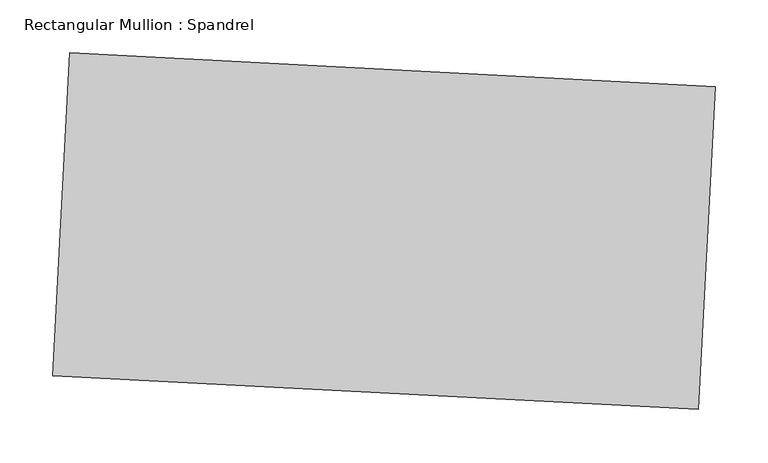
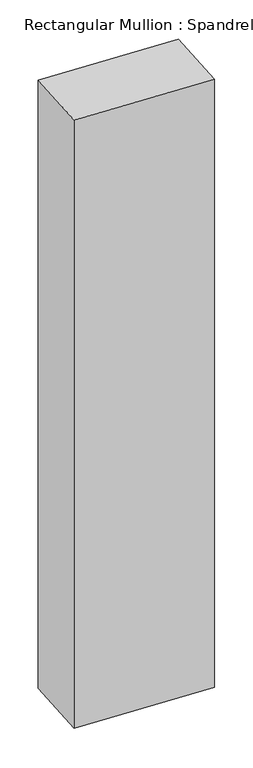
"""IFC4 building model written with IfcOpenShell, lengths in millimetres: member geometry, Rectangular Mullion : Spandrel."""

from ifc_helpers import new_model, si_unit, frame, origin, place, context, project, spatial, polyline, outline, extrude, source, transform, mapped, element, save


def rectangular_mullion_spandrel_2c0fee7e(model_context):
    return source(origin(), model_context, "Body", "SweptSolid", [
        extrude(outline(polyline([(7.5582819, 136.2391416), (-8.3937175, -168.1431406), (-617.1582819, -136.2391416), (-601.2062825, 168.1431406), (7.5582819, 136.2391416)])), frame((0.0, 0.0, -2875.2688367), z_axis=(0.0, 0.0, 1.0), x_axis=(1.0, 0.0, 0.0)), (0.0, 0.0, 1.0), 2875.2688367),
    ])


if __name__ == "__main__":
    model = new_model("IFC4")
    model_context = context("Model", 3, world=origin())
    ifc_project = project(units=[si_unit("LENGTHUNIT", "METRE", prefix="MILLI")], contexts=[model_context])
    site = spatial("IfcSite", under=ifc_project)
    building = spatial("IfcBuilding", under=site)
    placement = place(None, origin())
    rectangular_mullion_spandrel_shape = rectangular_mullion_spandrel_2c0fee7e(model_context)
    element("IfcMember", 1, ObjectType="Rectangular Mullion : Spandrel", at=placement, inside=building, context=model_context, shape_type="MappedRepresentation", body=[
        mapped(rectangular_mullion_spandrel_shape, transform((0.0, 0.0, 0.0), x_axis=(1.0, 0.0, 0.0), y_axis=(0.0, 1.0, 0.0), z_axis=(0.0, 0.0, 1.0))),
    ])
    save(model, "model.ifc")

# Revit data of these elements
# Type "Rectangular Mullion : Spandrel"
#   built-in parameter 1007304 = 1 (stored number, unit not read)
#   built-in parameter 1007301 = 1 (stored number, unit not read)
#   built-in parameter 1007300 = 1 (stored number, unit not read)
# Element 1 (IfcMember, "Rectangular Mullion : Spandrel")
#   Materials on its faces: "Aluminum"
# Materials
#   "Aluminum": class "Metal", colour RGB 247 247 247, transparency 0, Description = "Aluminum 6061", Cost = 0
